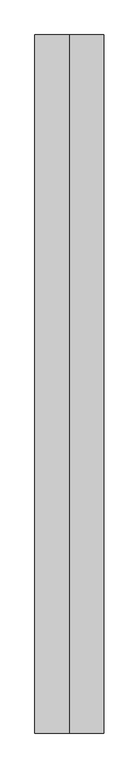
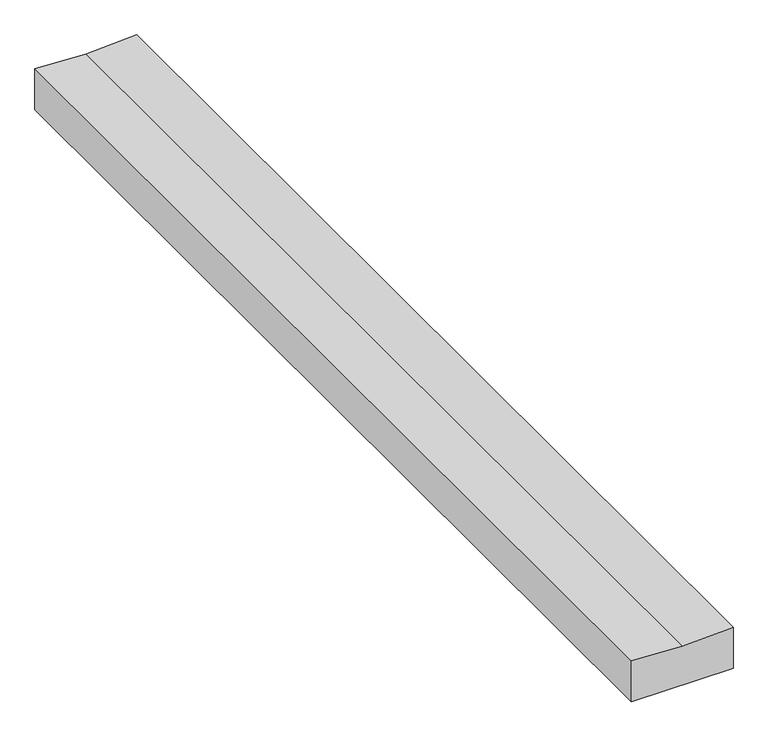
"""IFC4 building model written with IfcOpenShell, lengths in millimetres: proxy geometry, FIRESTONE INSULATION3:FIRESTONE INSULATION002:300188 : FIRESTONE INSULATION3:FIRESTONE INSULATION002:300188."""

from ifc_helpers import new_model, si_unit, frame, origin, place, context, project, spatial, polyline, outline, extrude, source, transform, mapped, element, save


def generic_models_7e8b6511(model_context):
    return source(origin(), model_context, "Body", "SweptSolid", [
        extrude(outline(polyline([(40216.0142809, -20.8947745), (40131.746, -20.8947745), (40131.746, 175.9552255), (40216.0142809, 175.9552255), (40211.0127094, 77.2027316), (40216.0142809, -20.8947745)])), frame((0.0, -774.3081162, 0.0), z_axis=(0.0, 1.0, 0.0), x_axis=(0.0, 0.0, 1.0)), (0.0, 0.0, 1.0), 2000.0),
    ])


if __name__ == "__main__":
    model = new_model("IFC4")
    model_context = context("Model", 3, world=origin())
    ifc_project = project(units=[si_unit("LENGTHUNIT", "METRE", prefix="MILLI")], contexts=[model_context])
    site = spatial("IfcSite", under=ifc_project)
    building = spatial("IfcBuilding", under=site)
    placement = place(None, origin())
    generic_models_shape = generic_models_7e8b6511(model_context)
    element("IfcBuildingElementProxy", 1, Name="FIRESTONE INSULATION3:FIRESTONE INSULATION002:300188 : FIRESTONE INSULATION3:FIRESTONE INSULATION002:300188", ObjectType="FIRESTONE INSULATION3:FIRESTONE INSULATION002:300188 : FIRESTONE INSULATION3:FIRESTONE INSULATION002:300188", at=placement, inside=building, context=model_context, shape_type="MappedRepresentation", body=[
        mapped(generic_models_shape, transform((0.0, 0.0, 0.0), x_axis=(1.0, 0.0, 0.0), y_axis=(0.0, 1.0, 0.0), z_axis=(0.0, 0.0, 1.0))),
    ])
    save(model, "model.ifc")

# Revit data of these elements
# Type "FIRESTONE INSULATION3:FIRESTONE INSULATION002:300188 : FIRESTONE INSULATION3:FIRESTONE INSULATION002:300188"
#   NameOverride = "FIRESTONE INSULATION3:FIRESTONE INSULATION002:300188"
#   ObjectTypeOverride = "FIRESTONE INSULATION3:FIRESTONE INSULATION002"
#   Reference = "FIRESTONE INSULATION002"
#   Category = "Generic Models"
#   Tag = "300188"
# Element 1 (IfcBuildingElementProxy, "FIRESTONE INSULATION3:FIRESTONE INSULATION002:300188 : FIRESTONE INSULATION3:FIRESTONE INSULATION002:300188")
#   Materials on its faces: "TAPERED 2X SLEEPERS - SLOPED TO DRAIN"
# Materials
#   "TAPERED 2X SLEEPERS - SLOPED TO DRAIN": class "Unassigned", colour RGB 234 198 178, transparency 0
